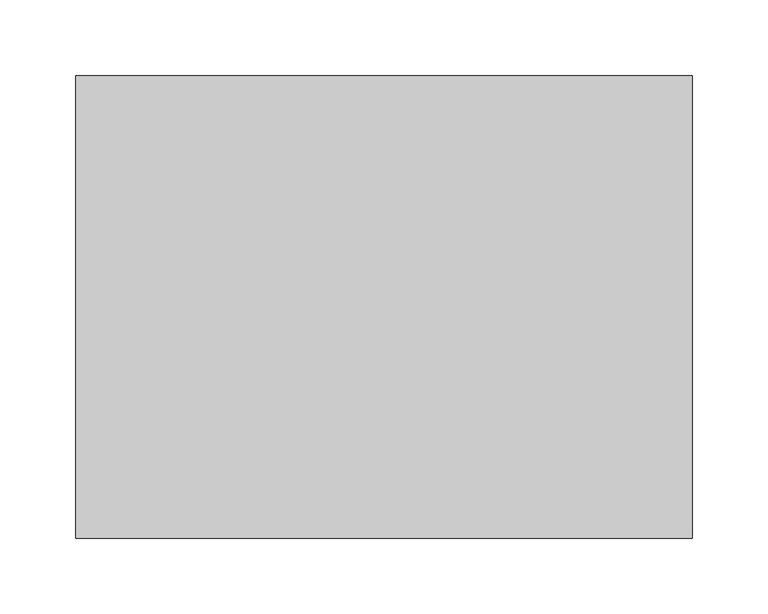
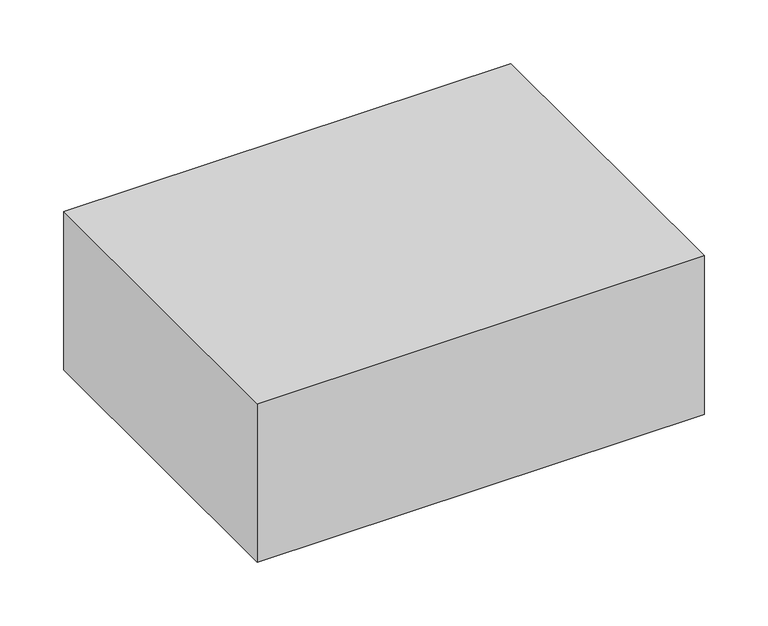
"""IFC4 building model written with IfcOpenShell, lengths in millimetres: proxy geometry, A1130 - Cabinet, Control, Nitrogen : A1130 - Cabinet, Control, Nitrogen."""

from ifc_helpers import new_model, si_unit, frame, origin, origin_with_axes, place, context, project, spatial, polyline, circle_curve, outline, extrude, faceted_brep, source, transform, mapped, element, save
from ifc_brep_helpers import plane_surface, cylinder_surface, advanced_brep


def specialty_equipment_5f64b538(model_context):
    return source(origin(), model_context, "Body", "SolidModel", [
        advanced_brep(
        [(-134.8279388, 159.2813257, 76.2), (-134.8279388, 146.5813257, 76.2), (-88.5288579, 146.5813257, 76.2), (-64.540234, 152.4, 76.2), (-87.9143784, 159.2813257, 76.2), (-134.8279388, 146.5813257, 58.4051365), (-134.8279388, 159.2813257, 58.4051365), (-87.9143784, 159.2813257, 58.4051365), (-89.940234, 152.4, 58.4051365), (-88.5288579, 146.5813257, 58.4051365), (-89.940234, 152.4, 25.4), (-64.540234, 152.4, 25.4)],
        [
            (0, 1),
            (1, 2),
            (2, 3, circle_curve(frame((-77.240234, 152.4, 76.2), z_axis=(0.0, 0.0, 1.0), x_axis=(1.0, 0.0, 0.0)), 12.7)),
            (3, 4, circle_curve(frame((-77.240234, 152.4, 76.2), z_axis=(0.0, 0.0, 1.0), x_axis=(1.0, 0.0, 0.0)), 12.7)),
            (4, 0),
            (5, 6),
            (6, 7),
            (7, 8, circle_curve(frame((-77.240234, 152.4, 58.4051365), z_axis=(0.0, 0.0, 1.0), x_axis=(1.0, 0.0, 0.0)), 12.7)),
            (8, 9, circle_curve(frame((-77.240234, 152.4, 58.4051365), z_axis=(0.0, 0.0, 1.0), x_axis=(1.0, 0.0, 0.0)), 12.7)),
            (9, 5),
            (0, 6),
            (5, 1),
            (9, 2),
            (4, 7),
            (10, 11, circle_curve(frame((-77.240234, 152.4, 25.4), z_axis=(0.0, 0.0, -1.0), x_axis=(1.0, 0.0, 0.0)), 12.7)),
            (11, 10, circle_curve(frame((-77.240234, 152.4, 25.4), z_axis=(0.0, 0.0, -1.0), x_axis=(1.0, 0.0, 0.0)), 12.7)),
            (11, 3),
            (8, 10),
        ],
        [
            plane_surface(frame((-134.8279388, 159.2813257, 76.2), z_axis=(0.0, 0.0, 1.0), x_axis=(0.0, -1.0, 0.0))),
            plane_surface(frame((-134.8279388, 159.2813257, 58.4051365), z_axis=(0.0, 0.0, -1.0), x_axis=(0.0, 1.0, 0.0))),
            plane_surface(frame((-134.8279388, 159.2813257, 76.2), z_axis=(-1.0, 0.0, 0.0), x_axis=(0.0, 0.0, -1.0))),
            plane_surface(frame((-134.8279388, 146.5813257, 76.2), z_axis=(0.0, -1.0, 0.0), x_axis=(0.0, 0.0, -1.0))),
            plane_surface(frame((-77.6779388, 159.2813257, 76.2), z_axis=(0.0, 1.0, 0.0), x_axis=(0.0, 0.0, -1.0))),
            plane_surface(frame((-64.540234, 152.4, 25.4), z_axis=(0.0, 0.0, -1.0), x_axis=(0.0, -1.0, 0.0))),
            cylinder_surface(frame((-77.240234, 152.4, 25.4), z_axis=(0.0, 0.0, 1.0), x_axis=(1.0, 0.0, 0.0)), 12.7),
        ],
        [
            (0, [[1, 2, 3, 4, 5]]),
            (1, [[6, 7, 8, 9, 10]]),
            (2, [[-1, 11, -6, 12]]),
            (3, [[-12, -10, 13, -2]]),
            (4, [[-11, -5, 14, -7]]),
            (5, [[15, 16]]),
            (6, [[-16, 17, -3, -13, -9, 18]]),
            (6, [[-15, -18, -8, -14, -4, -17]]),
        ],
    ),
        advanced_brep(
        [(19.6525292, 159.2813257, 76.2), (19.6525292, 146.5813257, 76.2), (65.9516102, 146.5813257, 76.2), (89.940234, 152.4, 76.2), (66.5660897, 159.2813257, 76.2), (19.6525292, 146.5813257, 58.4051365), (19.6525292, 159.2813257, 58.4051365), (66.5660897, 159.2813257, 58.4051365), (64.540234, 152.4, 58.4051365), (65.9516102, 146.5813257, 58.4051365), (64.540234, 152.4, 25.4), (89.940234, 152.4, 25.4)],
        [
            (0, 1),
            (1, 2),
            (2, 3, circle_curve(frame((77.240234, 152.4, 76.2), z_axis=(0.0, 0.0, 1.0), x_axis=(1.0, 0.0, 0.0)), 12.7)),
            (3, 4, circle_curve(frame((77.240234, 152.4, 76.2), z_axis=(0.0, 0.0, 1.0), x_axis=(1.0, 0.0, 0.0)), 12.7)),
            (4, 0),
            (5, 6),
            (6, 7),
            (7, 8, circle_curve(frame((77.240234, 152.4, 58.4051365), z_axis=(0.0, 0.0, 1.0), x_axis=(1.0, 0.0, 0.0)), 12.7)),
            (8, 9, circle_curve(frame((77.240234, 152.4, 58.4051365), z_axis=(0.0, 0.0, 1.0), x_axis=(1.0, 0.0, 0.0)), 12.7)),
            (9, 5),
            (0, 6),
            (5, 1),
            (9, 2),
            (4, 7),
            (10, 11, circle_curve(frame((77.240234, 152.4, 25.4), z_axis=(0.0, 0.0, -1.0), x_axis=(1.0, 0.0, 0.0)), 12.7)),
            (11, 10, circle_curve(frame((77.240234, 152.4, 25.4), z_axis=(0.0, 0.0, -1.0), x_axis=(1.0, 0.0, 0.0)), 12.7)),
            (11, 3),
            (8, 10),
        ],
        [
            plane_surface(frame((-134.8279388, 159.2813257, 76.2), z_axis=(0.0, 0.0, 1.0), x_axis=(0.0, -1.0, 0.0))),
            plane_surface(frame((-134.8279388, 159.2813257, 58.4051365), z_axis=(0.0, 0.0, -1.0), x_axis=(0.0, 1.0, 0.0))),
            plane_surface(frame((19.6525292, 159.2813257, 76.2), z_axis=(-1.0, 0.0, 0.0), x_axis=(0.0, 0.0, -1.0))),
            plane_surface(frame((19.6525292, 146.5813257, 76.2), z_axis=(0.0, -1.0, 0.0), x_axis=(0.0, 0.0, -1.0))),
            plane_surface(frame((76.8025292, 159.2813257, 76.2), z_axis=(0.0, 1.0, 0.0), x_axis=(0.0, 0.0, -1.0))),
            plane_surface(frame((-64.540234, 152.4, 25.4), z_axis=(0.0, 0.0, -1.0), x_axis=(0.0, -1.0, 0.0))),
            cylinder_surface(frame((77.240234, 152.4, -25.4), z_axis=(0.0, 0.0, 1.0), x_axis=(1.0, 0.0, 0.0)), 12.7),
        ],
        [
            (0, [[1, 2, 3, 4, 5]]),
            (1, [[6, 7, 8, 9, 10]]),
            (2, [[-1, 11, -6, 12]]),
            (3, [[-12, -10, 13, -2]]),
            (4, [[-11, -5, 14, -7]]),
            (5, [[15, 16]]),
            (6, [[-16, 17, -3, -13, -9, 18]]),
            (6, [[-15, -18, -8, -14, -4, -17]]),
        ],
    ),
        faceted_brep([(177.8, 266.7, 0.0), (-177.8, 266.7, 0.0), (-177.8, 266.7, 76.2), (177.8, 266.7, 76.2), (177.8, 38.1, 0.0), (177.8, 38.1, 76.2), (-177.8, 38.1, 76.2), (-177.8, 38.1, 0.0), (152.4, 63.5, 76.2), (-152.4, 63.5, 76.2), (-152.4, 241.3, 76.2), (152.4, 241.3, 76.2), (-152.4, 63.5, 25.4), (152.4, 63.5, 25.4), (152.4, 241.3, 25.4), (-152.4, 241.3, 25.4)], [[[0, 1, 2, 3]], [[4, 5, 6, 7]], [[1, 0, 4, 7]], [[2, 1, 7, 6]], [[3, 2, 6, 5], [8, 9, 10, 11]], [[0, 3, 5, 4]], [[12, 13, 14, 15]], [[13, 12, 9, 8]], [[14, 13, 8, 11]], [[15, 14, 11, 10]], [[12, 15, 10, 9]]]),
        extrude(outline(polyline([(203.2, 304.8), (203.2, 0.0), (-203.2, 0.0), (-203.2, 304.8), (203.2, 304.8)])), origin_with_axes(), (0.0, 0.0, 1.0), 152.4),
    ])


if __name__ == "__main__":
    model = new_model("IFC4")
    model_context = context("Model", 3, world=origin())
    ifc_project = project(units=[si_unit("LENGTHUNIT", "METRE", prefix="MILLI")], contexts=[model_context])
    site = spatial("IfcSite", under=ifc_project)
    building = spatial("IfcBuilding", under=site)
    placement = place(None, origin())
    specialty_equipment_shape = specialty_equipment_5f64b538(model_context)
    element("IfcBuildingElementProxy", 1, Name="A1130 - Cabinet, Control, Nitrogen : A1130 - Cabinet, Control, Nitrogen", ObjectType="A1130 - Cabinet, Control, Nitrogen : A1130 - Cabinet, Control, Nitrogen", at=placement, inside=building, context=model_context, shape_type="MappedRepresentation", body=[
        mapped(specialty_equipment_shape, transform((0.0, 0.0, 0.0), x_axis=(1.0, 0.0, 0.0), y_axis=(0.0, 1.0, 0.0), z_axis=(0.0, 0.0, 1.0))),
    ])
    save(model, "model.ifc")

# Revit data of these elements
# Type "A1130 - Cabinet, Control, Nitrogen : A1130 - Cabinet, Control, Nitrogen"
#   Watts2 = "0"
#   Watts1 = "0"
#   Unit_Issue = "EA"
#   UTIL_6_Misc = "-"
#   UTIL_5_NonMedGas = "-"
#   UTIL_4_MiscGas = "-"
#   UTIL_3_MedGas = "-"
#   UTIL_2_Elec = "B"
#   UTIL_1_WaterDrain = "-"
#   Nomenclature = "Cabinet, Control, Nitrogen"
#   NSN = "6530"
#   Location [instance default] = ""
#   JSN = "A1130"
#   Fund_Source_VA = "-"
#   Fund_Source_Navy = "-"
#   Fund_Source_Army = "-"
#   Fund_Source_AF = "-"
#   ELEC_Volts2 = "0"
#   ELEC_Volts1 = "0"
#   ELEC_Phase2 = "0"
#   ELEC_Phase1 = "0"
#   ELEC_HertzSwitch = "0"
#   ELEC_HertzDependent = "0"
#   ELEC_Hertz = "0"
#   ELEC_Amps2 = "0"
#   ELEC_Amps1 = "0"
#   DetailDescription = "Nitrogen control cabinet. Unit consists of supply cut-off valve, supply pressure gauge, pressure regulator (adjustable 0 to 200 PSI), outlet pressure gauge, nitrogen outlet and connection to surgical gas column. Specify recessed or surface mounting. Designed for powering surgical pneumatic tools."
#   CAT_VA = "A"
#   CAT_Navy = "A"
#   CAT_IHS = "-"
#   CAT_Army = "A"
#   CAT_AF = "A"
#   BTUperhour = "0"
#   Weight_IP = 10
#   Default Elevation = 3' - 7 1/2"
#   DIM_Width_IP = 1' - 4"
#   DIM_Height_IP = 1' - 0"
#   DIM_Depth_IP = 0' - 6"
#   Assembly Code = ""
# Element 1 (IfcBuildingElementProxy, "A1130 - Cabinet, Control, Nitrogen : A1130 - Cabinet, Control, Nitrogen")
#   Materials on its faces: "EquipSpace"
# Materials
#   "EquipSpace": class "Unassigned", colour RGB 221 217 195, transparency 0.5
